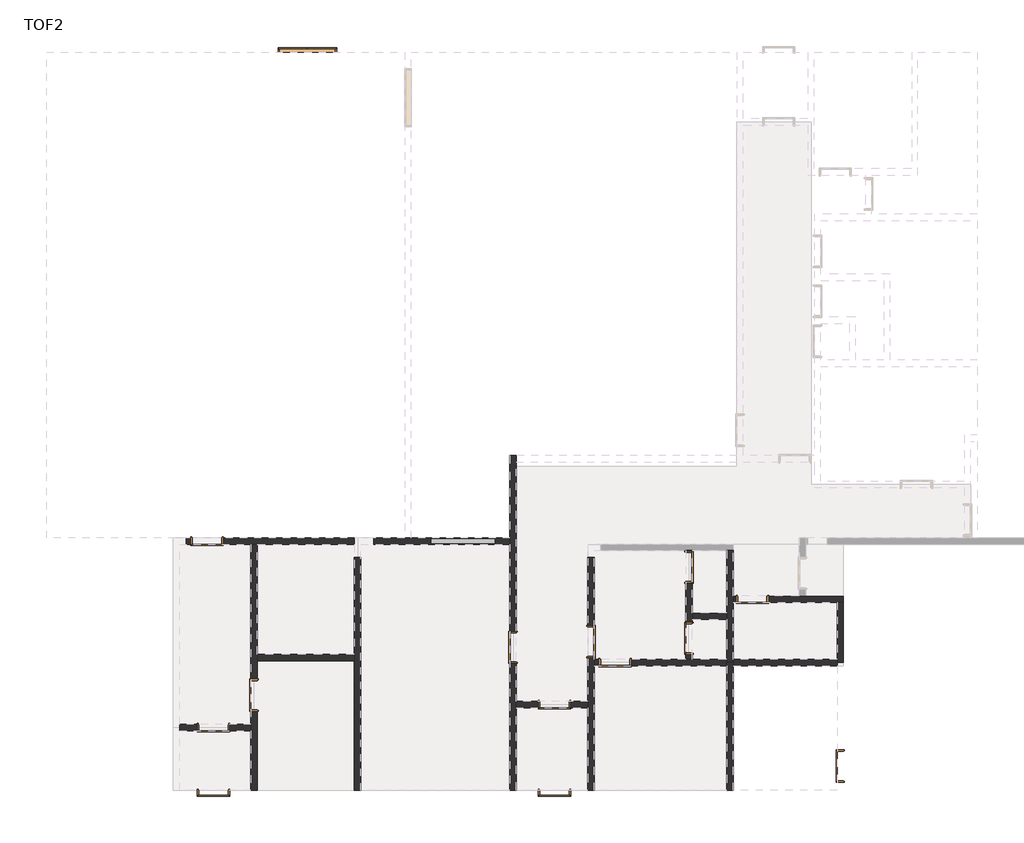
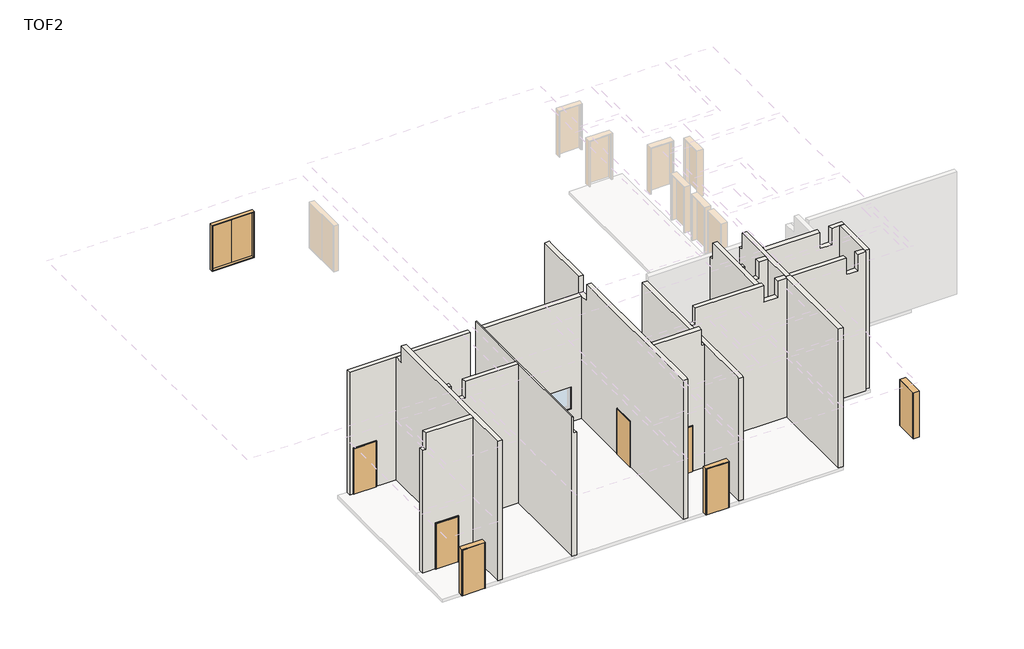
# One storey, part 1 of 2: 16 walls, 14 doors.
# Revit data of these elements (continued)
# Room at (43870, 7604.869) mm, phase "New Construction", upper level "TOC", upper offset 2000 mm, lower offset -2000 mm (continued)
#   H_Floor-Base Material-2 = "Steel Trowel Finish"
#   H_Floor-Base Material-3 = ""
#   H_Floor-Base Material-4 = ""
#   H_Floor-Base Material-5 = "Vinyl Tile"
#   H_Floor Finish-1 = "Vinyl Tile"
#   H_Floor Finish-2 = ""
#   H_Floor Finish Remark = ""
#   H_Skirt Base Material = "Same as Wall"
#   H_Skirt-Base Material-1 = ""
#   H_Skirt-Base Material-2 = ""
#   H_Skirt-Base Material-3 = ""
#   H_Skirt-Base Material-4 = ""
#   H_Skirt-Base Material-5 = ""
#   H_Skirt Finish-1 = "Vinyl Tile"
#   H_Skirt Finish-2 = ""
#   H_Skirt Finish Remark = "Vinyl Tile = PVC Tile (polyvinyl chloride)"
#   H_Wall Finish Style Name = "Acrylic Emulsion Paint"
#   H_Wall Base Material = "Masonry Wall / Cement Plaster"
#   H_Wall-Base Material-4 = ""
#   H_Wall-Base Material-5 = ""
#   H_Wall Finish-1 = "Acrylic Emulsion Paint"
#   H_Wall Finish-2 = ""
#   H_Wall Finish Remark = "T13 Plaster"
#   H_Ceiling Finish Style Name = "Suspended Acoustic Tiled Ceiling (M-Bar)"
#   H_Ceiling Base Material = "Concrete Slab / Fair Faced Concrete"
#   H_Ceiling-Base Material-1 = "(Concrete Slab)"
#   H_Ceiling-Base Material-2 = "(Fair Faced Concrete)"
#   H_Ceiling-Base Material-3 = ""
#   H_Ceiling-Base Material-4 = ""
#   H_Ceiling-Base Material-5 = "Acoustic Tiled Ceiling System (M-Bar)"
#   H_Ceiling Finish-1 = "Acoustic Tiled Ceiling System (M-Bar)"
#   H_Ceiling Finish-2 = ""
#   H_Ceiling Finish Remark = ""
#   Floor Finish Style No = F34A
#   Skirt Finish Style No = B35
#   Wall Finish Style No = W01B
#   Ceiling Finish Style No = C95A
# Room at (37870, 1977.173) mm, phase "New Construction", upper level "TOC", upper offset 2000 mm, lower offset -2000 mm
#   Comments = ""
#   Number = "119"
#   Name = "AIR LOCK"
#   H_Floor Finish Style Name = "Vinyl Tile"
#   H_Floor Base Material = "Concrete Slab / Steel Trowel Finish"
#   H_Wall-Base Material-1 = "Masonry Wall"
#   H_Skirt Finish Style Name = "Coved Vinyl Tile"
#   H_Wall-Base Material-2 = ""
#   H_Wall-Base Material-3 = "Plastering"
#   H_Floor-Base Material-1 = "Concrete Slab"
#   H_Floor-Base Material-2 = "Steel Trowel Finish"
#   H_Floor-Base Material-3 = ""
#   H_Floor-Base Material-4 = ""
#   H_Floor-Base Material-5 = "Vinyl Tile"
#   H_Floor Finish-1 = "Vinyl Tile"
#   H_Floor Finish-2 = ""
#   H_Floor Finish Remark = ""
#   H_Skirt Base Material = "Same as Wall"
#   H_Skirt-Base Material-1 = ""
#   H_Skirt-Base Material-2 = ""
#   H_Skirt-Base Material-3 = ""
#   H_Skirt-Base Material-4 = ""
#   H_Skirt-Base Material-5 = ""
#   H_Skirt Finish-1 = "Vinyl Tile"
#   H_Skirt Finish-2 = ""
#   H_Skirt Finish Remark = "Vinyl Tile = PVC Tile (polyvinyl chloride)"
#   H_Wall Finish Style Name = "Acrylic Emulsion Paint"
#   H_Wall Base Material = "Masonry Wall / Cement Plaster"
#   H_Wall-Base Material-4 = ""
#   H_Wall-Base Material-5 = ""
#   H_Wall Finish-1 = "Acrylic Emulsion Paint"
#   H_Wall Finish-2 = ""
#   H_Wall Finish Remark = "T13 Plaster"
#   H_Ceiling Finish Style Name = "Suspended Acoustic Tiled Ceiling (M-Bar)"
#   H_Ceiling Base Material = "Concrete Slab / Fair Faced Concrete"
#   H_Ceiling-Base Material-1 = "(Concrete Slab)"
#   H_Ceiling-Base Material-2 = "(Fair Faced Concrete)"
#   H_Ceiling-Base Material-3 = ""
#   H_Ceiling-Base Material-4 = ""
#   H_Ceiling-Base Material-5 = "Acoustic Tiled Ceiling System (M-Bar)"
#   H_Ceiling Finish-1 = "Acoustic Tiled Ceiling System (M-Bar)"
#   H_Ceiling Finish-2 = ""
#   H_Ceiling Finish Remark = ""
#   Floor Finish Style No = F34A
#   Skirt Finish Style No = B35
#   Wall Finish Style No = W01B
#   Ceiling Finish Style No = C95A
